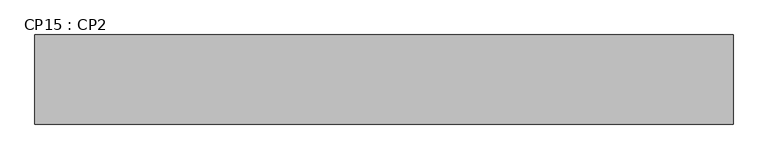
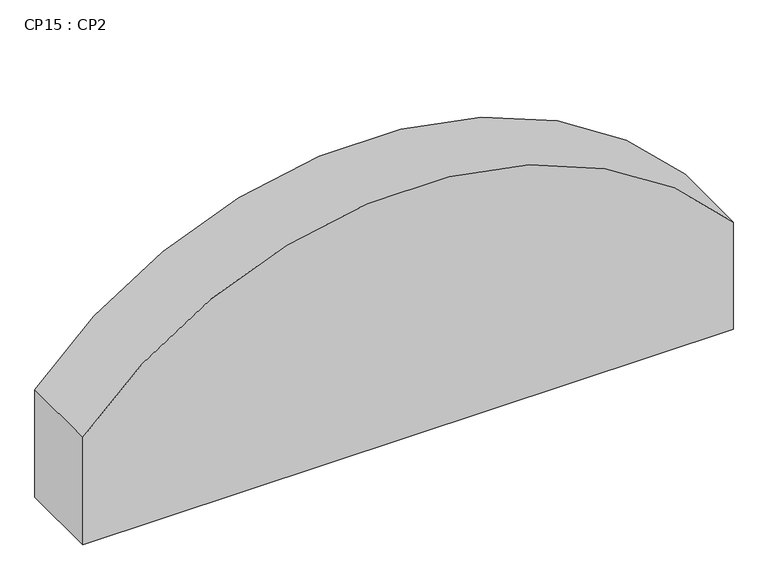
"""IFC4 building model written with IfcOpenShell, lengths in millimetres: beam geometry, CP15 : CP2."""

from ifc_helpers import new_model, si_unit, frame, origin, place, context, project, spatial, circle_curve, source, transform, mapped, element, save
from ifc_brep_helpers import plane_surface, cylinder_surface, advanced_brep


def cp15_cp2_57de0c29(model_context):
    return source(origin(), model_context, "Body", "AdvancedBrep", [
        advanced_brep(
        [(19843.224554, 19499.7448212, 14620.0), (15143.2245541, 19499.7448212, 14620.0), (15143.2245527, 19499.7448212, 13800.0), (19843.2245533, 19499.7448212, 13800.0), (15143.2245527, 20099.7448193, 13800.0), (15143.2245527, 20099.7448193, 14620.0), (19843.224554, 20099.7448193, 14620.0), (19843.2245533, 20099.7448193, 13800.0)],
        [
            (0, 1, circle_curve(frame((17493.224554, 19499.7448212, 12603.8185575), z_axis=(0.0, -1.0, 0.0), x_axis=(0.0, 0.0, -1.0)), 3096.3668402)),
            (1, 2),
            (2, 3),
            (3, 0),
            (4, 5),
            (5, 6, circle_curve(frame((17493.224554, 20099.7448193, 12603.8185575), z_axis=(0.0, 1.0, 0.0), x_axis=(0.0, 0.0, -1.0)), 3096.3668402)),
            (6, 7),
            (7, 4),
            (2, 4),
            (7, 3),
            (0, 6),
            (5, 1),
        ],
        [
            plane_surface(frame((19993.2245542, 19499.7448212, 13800.0), z_axis=(0.0, -1.0, 0.0), x_axis=(0.0, 0.0, 1.0))),
            plane_surface(frame((19993.2245542, 20099.7448193, 13800.0), z_axis=(0.0, 1.0, 0.0), x_axis=(0.0, 0.0, -1.0))),
            plane_surface(frame((14993.2245543, 19499.7448212, 13800.0), z_axis=(0.0, 0.0, -1.0), x_axis=(0.0, 1.0, 0.0))),
            cylinder_surface(frame((17493.224554, 20099.7448193, 12603.8185575), z_axis=(0.0, 1.0, 0.0), x_axis=(0.0, 0.0, -1.0)), 3096.3668402),
            plane_surface(frame((15143.2245527, 18587.0448193, 14620.0), z_axis=(-1.0, 0.0, 0.0), x_axis=(0.0, -1.0, 0.0))),
            plane_surface(frame((19843.2245533, 18587.0448193, 13800.0), z_axis=(1.0, 0.0, 0.0), x_axis=(0.0, -1.0, 0.0))),
        ],
        [
            (0, [[1, 2, 3, 4]]),
            (1, [[5, 6, 7, 8]]),
            (2, [[9, -8, 10, -3]]),
            (3, [[-1, 11, -6, 12]]),
            (4, [[-2, -12, -5, -9]]),
            (5, [[-4, -10, -7, -11]]),
        ],
    ),
    ])


if __name__ == "__main__":
    model = new_model("IFC4")
    model_context = context("Model", 3, world=origin())
    ifc_project = project(units=[si_unit("LENGTHUNIT", "METRE", prefix="MILLI")], contexts=[model_context])
    site = spatial("IfcSite", under=ifc_project)
    building = spatial("IfcBuilding", under=site)
    placement = place(None, origin())
    cp15_cp2_shape = cp15_cp2_57de0c29(model_context)
    element("IfcBeam", 1, ObjectType="CP15 : CP2", at=placement, inside=building, context=model_context, shape_type="MappedRepresentation", body=[
        mapped(cp15_cp2_shape, transform((0.0, 0.0, 0.0), x_axis=(1.0, 0.0, 0.0), y_axis=(0.0, 1.0, 0.0), z_axis=(0.0, 0.0, 1.0))),
    ])
    save(model, "model.ifc")
